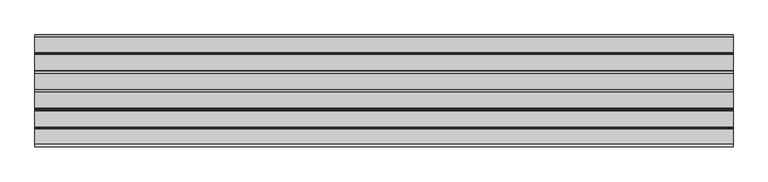
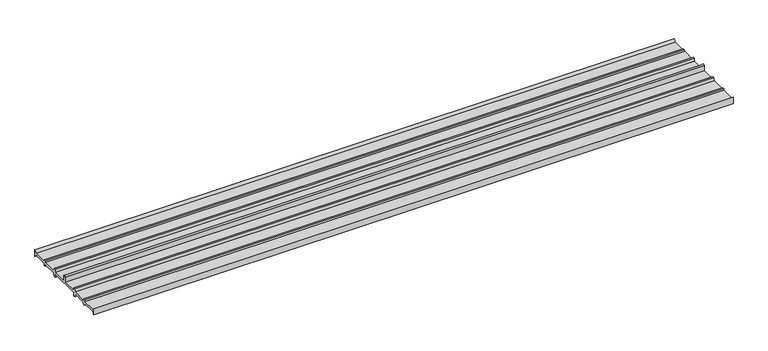
"""IFC4 building model written with IfcOpenShell, lengths in millimetres: proxy geometry, TN_ПВХ_ТПО_Гидрошпонка ТехноНИКОЛЬ : ПВХ Гидрошпонка ТехноНИКОЛЬ IC-240-6."""

from ifc_helpers import new_model, si_unit, point, frame, frame_2d, origin, place, context, project, spatial, polyline, circle_curve, trimmed, segment, composite_curve, outline, extrude, source, transform, mapped, element, save


def specialty_equipment_90407aac(model_context):
    return source(origin(), model_context, "Body", "SweptSolid", [
        extrude(outline(composite_curve([segment(polyline([(36.8860421, 0.0), (-36.8860421, 0.0), (-38.1581338, -7.7258715), (-41.8418662, -7.7258715), (-43.1139579, 0.0), (-77.2655559, 0.0), (-78.1337968, -4.9240388), (-81.8662032, -4.9240388), (-82.7344441, 0.0), (-114.7630952, 0.0), (-120.0, -5.2369048), (-120.0, 10.2369048), (-114.7630952, 5.0), (-82.5038474, 5.0), (-81.8662032, 8.8726426), (-78.1337968, 8.8726426), (-77.4969835, 5.0), (-42.9944406, 5.0), (-41.8418662, 12.0), (-38.1581338, 12.0), (-37.0055594, 5.0), (-2.5, 5.0), (-2.5, 17.5)]), True, "CONTINUOUS"), segment(trimmed(circle_curve(frame_2d((0.0, 17.5)), 2.5), [point((-2.5, 17.5))], [point((2.5, 17.5))], False, "CARTESIAN"), True, "CONTINUOUS"), segment(polyline([(2.5, 17.5), (2.5, 5.0), (37.0055594, 5.0), (38.1581338, 12.0), (41.8418662, 12.0), (42.9944406, 5.0), (77.4969835, 5.0), (78.1337968, 8.8726426), (81.8662032, 8.8726426), (82.5038474, 5.0), (114.7630952, 5.0), (120.0, 10.2369048), (120.0, -5.2369048), (114.7630952, 0.0), (82.7344441, 0.0), (81.8662032, -4.9240388), (78.1337968, -4.9240388), (77.2655559, 0.0), (43.1139579, 0.0), (41.8418662, -7.7258715), (38.1581338, -7.7258715), (36.8860421, 0.0)]), True, "CONTINUOUS")], self_intersect=False)), frame((0.0, 0.0, 0.0), z_axis=(1.0, 0.0, 0.0), x_axis=(0.0, 1.0, 0.0)), (0.0, 0.0, 1.0), 1500.0),
    ])


if __name__ == "__main__":
    model = new_model("IFC4")
    model_context = context("Model", 3, world=origin())
    ifc_project = project(units=[si_unit("LENGTHUNIT", "METRE", prefix="MILLI")], contexts=[model_context])
    site = spatial("IfcSite", under=ifc_project)
    building = spatial("IfcBuilding", under=site)
    placement = place(None, origin())
    specialty_equipment_shape = specialty_equipment_90407aac(model_context)
    element("IfcBuildingElementProxy", 1, Name="TN_ПВХ_ТПО_Гидрошпонка ТехноНИКОЛЬ : ПВХ Гидрошпонка ТехноНИКОЛЬ IC-240-6", ObjectType="TN_ПВХ_ТПО_Гидрошпонка ТехноНИКОЛЬ : ПВХ Гидрошпонка ТехноНИКОЛЬ IC-240-6", at=placement, inside=building, context=model_context, shape_type="MappedRepresentation", body=[
        mapped(specialty_equipment_shape, transform((0.0, 0.0, 0.0), x_axis=(1.0, 0.0, 0.0), y_axis=(0.0, 1.0, 0.0), z_axis=(0.0, 0.0, 1.0))),
    ])
    save(model, "model.ifc")

# Revit data of these elements
# Type "TN_ПВХ_ТПО_Гидрошпонка ТехноНИКОЛЬ : ПВХ Гидрошпонка ТехноНИКОЛЬ IC-240-6"
#   Description = "Внутренняя гидрошпонка для герметизации рабочих швов бетонирования в монолитных конструкциях при новом строительстве - подземных частей зданий, подземных парковок, тоннелей, коллекторов, дамб, каналов, резервуаров, бассейнов, очистных сооружений и пр."
#   Type Comments = "п.м."
#   Manufacturer = "ТехноНИКОЛЬ"
#   URL = "https://www.tstn.ru/product/pvkh-gidroshponka-tekhnonikol-ic-240-6-499185/"
#   ADSK_Примечание = ""
#   ADSK_Обозначение [instance default] = "ТехноНИКОЛЬ"
#   ADSK_Наименование = "ПВХ Гидрошпонка ТехноНИКОЛЬ IC-240-6"
#   ADSK_Масса_Текст = ""
#   ADSK_Марка = ""
#   ADSK_Код изделия = "499185"
#   ADSK_Завод-изготовитель [instance default] = "ТехноНИКОЛЬ"
#   ADSK_Единица измерения [instance default] = "п.м."
#   ADSK_Группирование = "Гидрошпонки"
#   ADSK_URL страницы изделия = "https://www.tstn.ru/product/pvkh-gidroshponka-tekhnonikol-ic-240-6-499185/"
#   ADSK_URL документации изделия = "https://nav.tn.ru/upload/iblock/67f/Katalog-i-rekomendatsii-po-primeneniyu_Gidroshponki-TEKHNONIKOL.PDF"
#   built-in parameter 1001306 [instance default] = 3.28084 (stored number, unit not read)
#   ADSK_Размер_Длина [instance default] = 1000 mm
#   ADSK_Количество [instance default] = 1
#   ПВХ_ТПО Гидрошпонка ТехноНИКОЛЬ EC-320-4 = no
#   ПВХ Гидрошпонка ТехноНИКОЛЬ IM-260/50 = no
#   ПВХ Гидрошпонка ТехноНИКОЛЬ IM-240/20 = no
#   ПВХ Гидрошпонка ТехноНИКОЛЬ IC-240-6 = yes
#   ПВХ Гидрошпонка ТехноНИКОЛЬ IC-125-2SP = no
#   ПВХ Гидрошпонка ТехноНИКОЛЬ EM-260/50 = no
#   ПВХ Гидрошпонка ТехноНИКОЛЬ EM-260/20 = no
#   ПВХ Гидрошпонка ТехноНИКОЛЬ EC-320-4 = no
#   ПВХ Гидрошпонка ТехноНИКОЛЬ EC-220-3 = no
#   ПВХ_ТПО Гидрошпонка ТехноНИКОЛЬ EC-220-3 = no
#   ПВХ Гидрошпонка ТехноНИКОЛЬ IC-240-2 = no
#   Материал = TN_ПВХ_Черный
#   Default Elevation = 0
# Element 1 (IfcBuildingElementProxy, "TN_ПВХ_ТПО_Гидрошпонка ТехноНИКОЛЬ : ПВХ Гидрошпонка ТехноНИКОЛЬ IC-240-6")
#   built-in parameter 1001306 = 4.92126 (stored number, unit not read)
#   ADSK_Размер_Длина = 1500 mm
#   ADSK_Количество = 1.5
#   Materials on its faces: "TN_ПВХ_Черный"
# Materials
#   "TN_ПВХ_Черный": class "Типовые", colour RGB 48 48 48, transparency 0, Cost = 0
